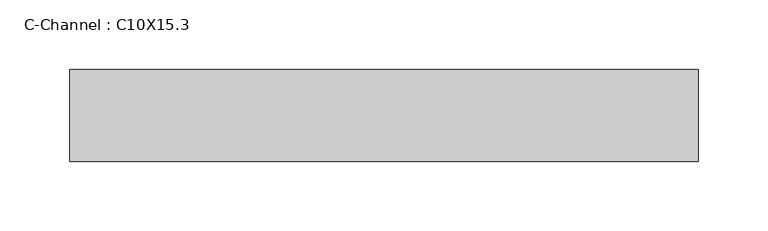
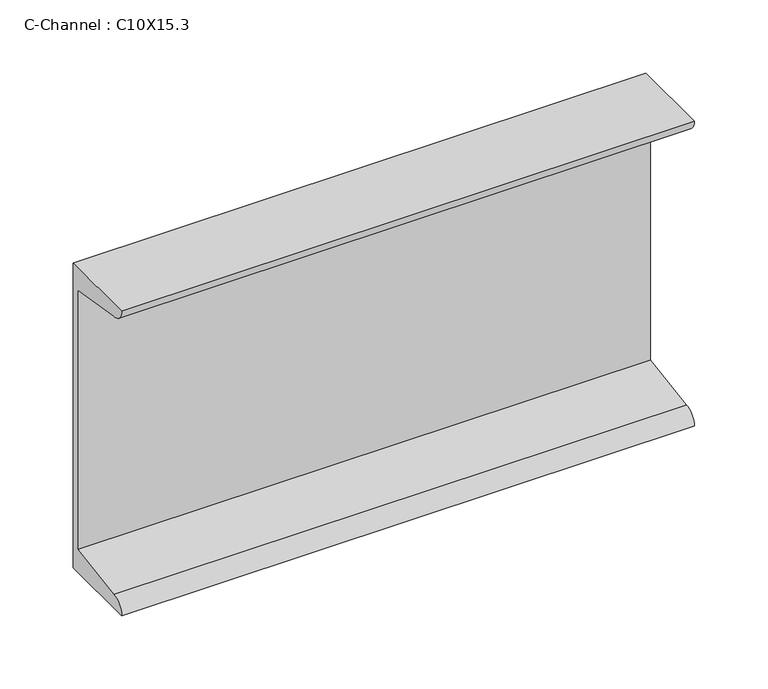
"""IFC4 building model written with IfcOpenShell, lengths in millimetres: beam geometry, C-Channel : C10X15.3."""

from ifc_helpers import new_model, si_unit, point, frame, frame_2d, origin, place, context, project, spatial, polyline, circle_curve, trimmed, segment, composite_curve, outline, extrude, source, transform, mapped, element, save


def c_channel_c10x15_3_fd865537(model_context):
    return source(origin(), model_context, "Body", "SweptSolid", [
        extrude(outline(composite_curve([segment(polyline([(16.1036, 127.0), (16.1036, -127.0), (-49.9364, -127.0)]), True, "CONTINUOUS"), segment(trimmed(circle_curve(frame_2d((-38.862, -127.0)), 11.0744), [point((-49.9364, -127.0))], [point((-38.862, -115.9256))], False, "CARTESIAN"), True, "CONTINUOUS"), segment(polyline([(-38.862, -115.9256), (10.0076, -108.1854158), (10.0076, 108.1854158), (-38.862, 115.9256)]), True, "CONTINUOUS"), segment(trimmed(circle_curve(frame_2d((-38.862, 127.0)), 11.0744), [point((-38.862, 115.9256))], [point((-49.9364, 127.0))], False, "CARTESIAN"), True, "CONTINUOUS"), segment(polyline([(-49.9364, 127.0), (16.1036, 127.0)]), True, "CONTINUOUS")], self_intersect=False)), frame((-178.308, 0.0, 0.0), z_axis=(1.0, 0.0, 0.0), x_axis=(0.0, 1.0, 0.0)), (0.0, 0.0, 1.0), 451.358),
    ])


if __name__ == "__main__":
    model = new_model("IFC4")
    model_context = context("Model", 3, world=origin())
    ifc_project = project(units=[si_unit("LENGTHUNIT", "METRE", prefix="MILLI")], contexts=[model_context])
    site = spatial("IfcSite", under=ifc_project)
    building = spatial("IfcBuilding", under=site)
    placement = place(None, origin())
    c_channel_c10x15_3_shape = c_channel_c10x15_3_fd865537(model_context)
    element("IfcBeam", 1, ObjectType="C-Channel : C10X15.3", at=placement, inside=building, context=model_context, shape_type="MappedRepresentation", body=[
        mapped(c_channel_c10x15_3_shape, transform((0.0, 0.0, 0.0), x_axis=(1.0, 0.0, 0.0), y_axis=(0.0, 1.0, 0.0), z_axis=(0.0, 0.0, 1.0))),
    ])
    save(model, "model.ifc")

# Revit data of these elements
# Type "C-Channel : C10X15.3"
#   Assembly Code = "B10"
#   W = 15.3
#   Length [instance default] = 5' - 0"
#   bf = 0' - 2.6"
#   d = 0' - 10"
#   tf = 0' - 0.436"
#   tw = 0' - 0.24"
#   x = 0' - 0.634"
#   A = 0.0311111 SF
#   Structural Material [instance default] = Steel ASTM A36
# Element 1 (IfcBeam, "C-Channel : C10X15.3")
#   Structural Material = Steel ASTM A992
#   Materials on its faces: "Steel ASTM A992"
# Materials
#   "Steel ASTM A36": class "Metal", colour RGB 199 199 199, transparency 0, Description = "Structural steel, ASTM A36 Grade B, mill finish", Cost = 0
#   "Steel ASTM A992": class "Metal", colour RGB 199 199 199, transparency 0, Description = "Structural steel 50ksi", Cost = 0
